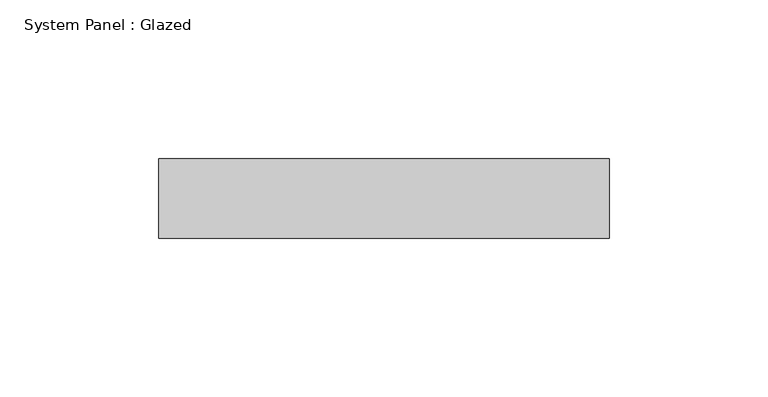
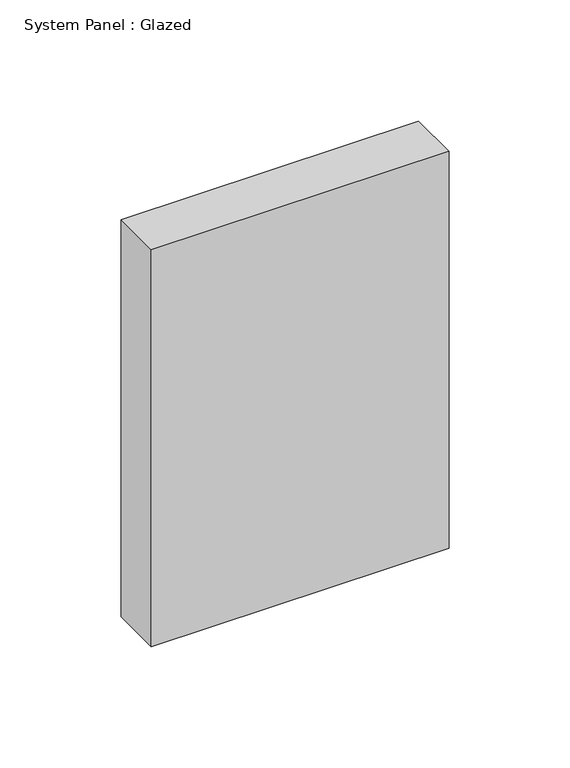
"""IFC4 building model written with IfcOpenShell, lengths in millimetres: plate geometry, System Panel : Glazed."""

import ifcopenshell
import ifcopenshell.guid

model = None  # the IFC model being written
_history = None  # IfcOwnerHistory: only IFC2X3 demands one
_inside = {}  # id of a spatial element -> (the spatial element, [elements in it])
_under = {}  # id of a project, library or spatial element -> (it, [spatial elements below it])
_declared = {}  # id of a project -> (the project, [libraries it declares])
_typed = {}  # id of a type object -> (the type object, [elements of that type])
_made_of = {}  # id of a material, layer set ... -> (it, [elements and type objects made of it])


def new_model(schema):
    """Start an empty IFC model of exactly this schema.

    Asked for "IFC4X3", IfcOpenShell would pick the latest addendum, in which some entities
    have other attributes; the version numbers below select the first issue.
    IFC2X3 requires an IfcOwnerHistory on every rooted entity: one is made here for all.
    """
    global model, _history
    if schema == "IFC4X3":
        model = ifcopenshell.file(schema_version=(4, 3, 0, 0))
    else:
        model = ifcopenshell.file(schema=schema)
    _inside.clear()
    _under.clear()
    _declared.clear()
    _typed.clear()
    _made_of.clear()
    _history = None
    if model.schema == "IFC2X3":
        org = make("IfcOrganization", Name="unknown")
        user = make(
            "IfcPersonAndOrganization",
            ThePerson=make("IfcPerson", FamilyName="unknown"),
            TheOrganization=org,
        )
        app = make(
            "IfcApplication",
            ApplicationDeveloper=org,
            Version="unknown",
            ApplicationFullName="unknown",
            ApplicationIdentifier="unknown",
        )
        _history = make(
            "IfcOwnerHistory",
            OwningUser=user,
            OwningApplication=app,
            ChangeAction="ADDED",
            CreationDate=0,
        )
    return model


def make(cls, **values):
    """One entity of the class cls with the attributes given. An attribute that is None is left unset."""
    return model.create_entity(
        cls, **{name: value for name, value in values.items() if value is not None}
    )


def rooted(cls, **values):
    """An entity with a GlobalId (a new one), such as an element, a storey or a relation."""
    return make(cls, GlobalId=ifcopenshell.guid.new(), OwnerHistory=_history, **values)


def si_unit(unit_type, name, prefix=None):
    """IfcSIUnit, for example si_unit("LENGTHUNIT", "METRE", prefix="MILLI")."""
    return make("IfcSIUnit", UnitType=unit_type, Prefix=prefix, Name=name)


def assignment(units):
    """IfcUnitAssignment: the units of a project."""
    return None if units is None else make("IfcUnitAssignment", Units=units)


def point(xyz):
    """IfcCartesianPoint."""
    return None if xyz is None else make("IfcCartesianPoint", Coordinates=xyz)


def direction(xyz):
    """IfcDirection."""
    return None if xyz is None else make("IfcDirection", DirectionRatios=xyz)


def frame(location, z_axis=None, x_axis=None):
    """IfcAxis2Placement3D, a coordinate frame: its origin and axes. An axis left out is left unset."""
    return make(
        "IfcAxis2Placement3D",
        Location=point(location),
        Axis=direction(z_axis),
        RefDirection=direction(x_axis),
    )


def origin():
    """The frame at (0, 0, 0) with its axes left unset."""
    return frame((0.0, 0.0, 0.0))


def origin_with_axes():
    """The frame at (0, 0, 0) with the z axis (0, 0, 1) and the x axis (1, 0, 0) written out."""
    return frame((0.0, 0.0, 0.0), z_axis=(0.0, 0.0, 1.0), x_axis=(1.0, 0.0, 0.0))


def place(relative_to, where):
    """IfcLocalPlacement: puts the frame where relative to a parent placement (None: the world)."""
    return make(
        "IfcLocalPlacement", PlacementRelTo=relative_to, RelativePlacement=where
    )


def context(
    kind, dimensions, precision=None, world=None, true_north=None, identifier=None
):
    """IfcGeometricRepresentationContext, for example the 3D "Model" context."""
    return make(
        "IfcGeometricRepresentationContext",
        ContextIdentifier=identifier,
        ContextType=kind,
        CoordinateSpaceDimension=dimensions,
        Precision=precision,
        WorldCoordinateSystem=world,
        TrueNorth=true_north,
    )


def project(units=None, contexts=None):
    """IfcProject with its units and contexts."""
    return rooted(
        "IfcProject",
        Name="project",
        RepresentationContexts=contexts,
        UnitsInContext=assignment(units),
    )


def spatial(cls, under=None, at=None, **own):
    """A site, building, storey or space (cls), placed at a placement, below another one or the project."""
    s = rooted(cls, ObjectPlacement=at, **own)
    if under is not None:
        _under.setdefault(under.id(), (under, []))[1].append(s)
    return s


def polyline(points):
    """IfcPolyline through the points."""
    return make("IfcPolyline", Points=[point(p) for p in points])


def outline(outer, holes=None, kind="AREA"):
    """IfcArbitraryClosedProfileDef: a profile drawn as a closed curve; with holes, ...WithVoids."""
    if holes is None:
        return make("IfcArbitraryClosedProfileDef", ProfileType=kind, OuterCurve=outer)
    return make(
        "IfcArbitraryProfileDefWithVoids",
        ProfileType=kind,
        OuterCurve=outer,
        InnerCurves=holes,
    )


def extrude(swept, where, along, depth):
    """IfcExtrudedAreaSolid: the profile swept, set in the frame where, extruded along a direction by depth."""
    return make(
        "IfcExtrudedAreaSolid",
        SweptArea=swept,
        Position=where,
        ExtrudedDirection=direction(along),
        Depth=depth,
    )


def shape(context_of_items, identifier, shape_type, items):
    """IfcShapeRepresentation: the items that make up one representation, for example the "Body"."""
    return make(
        "IfcShapeRepresentation",
        ContextOfItems=context_of_items,
        RepresentationIdentifier=identifier,
        RepresentationType=shape_type,
        Items=items,
    )


def source(mapping_origin, context_of_items, identifier, shape_type, items):
    """IfcRepresentationMap: a shape defined once, which mapped items show again and again."""
    return make(
        "IfcRepresentationMap",
        MappingOrigin=mapping_origin,
        MappedRepresentation=shape(context_of_items, identifier, shape_type, items),
    )


def transform(
    local_origin,
    x_axis=None,
    y_axis=None,
    z_axis=None,
    scale=None,
    scale2=None,
    scale3=None,
    uniform=True,
):
    """IfcCartesianTransformationOperator3D, or its non-uniform kind. x_axis, y_axis, z_axis: its Axis1, 2, 3."""
    if uniform:
        return make(
            "IfcCartesianTransformationOperator3D",
            Axis1=direction(x_axis),
            Axis2=direction(y_axis),
            LocalOrigin=point(local_origin),
            Scale=scale,
            Axis3=direction(z_axis),
        )
    return make(
        "IfcCartesianTransformationOperator3DnonUniform",
        Axis1=direction(x_axis),
        Axis2=direction(y_axis),
        LocalOrigin=point(local_origin),
        Scale=scale,
        Axis3=direction(z_axis),
        Scale2=scale2,
        Scale3=scale3,
    )


def mapped(mapping_source, mapping_target):
    """IfcMappedItem: shows the shape of a source again, moved by a transform."""
    return make(
        "IfcMappedItem", MappingSource=mapping_source, MappingTarget=mapping_target
    )


def made_of(thing, what):
    """Note that an element or type object is made of a material, layer set ...; save() writes the relation."""
    if what is not None:
        _made_of.setdefault(what.id(), (what, []))[1].append(thing)
    return thing


def element(
    cls,
    number,
    at=None,
    inside=None,
    cuts=None,
    type_object=None,
    material=None,
    context=None,
    identifier="Body",
    shape_type=None,
    held_by="IfcProductDefinitionShape",
    body=None,
    shapes=None,
    **own,
):
    """One element of the class cls, such as IfcWall. Its Tag is "e" and its number.

    at: its placement. inside: the storey or other place that contains it. cuts: it is an
    opening in that element (IfcRelVoidsElement). A single representation is given by context,
    identifier, shape_type and body (its items); several are given by shapes. held_by: the class
    of the entity that holds the representations. save() writes the other relations.
    """
    e = rooted(cls, Tag="e%d" % number, ObjectPlacement=at, **own)
    if body is not None:
        shapes = [shape(context, identifier, shape_type, body)]
    if shapes is not None:
        e.Representation = make(held_by, Representations=shapes)
    if inside is not None:
        _inside.setdefault(inside.id(), (inside, []))[1].append(e)
    if cuts is not None:
        rooted(
            "IfcRelVoidsElement", RelatingBuildingElement=cuts, RelatedOpeningElement=e
        )
    if type_object is not None:
        _typed.setdefault(type_object.id(), (type_object, []))[1].append(e)
    return made_of(e, material)


def aggregate(whole, parts):
    """IfcRelAggregates: a whole, such as a stair, and the parts it consists of."""
    return rooted("IfcRelAggregates", RelatingObject=whole, RelatedObjects=parts)


def save(model, path):
    """Write the relations noted so far, then the file.

    IfcRelAggregates (storeys below a building ...), IfcRelContainedInSpatialStructure (elements
    in a storey), IfcRelDefinesByType, IfcRelAssociatesMaterial and IfcRelDeclares: one each for
    every whole, place, type object, material and project.
    """
    for whole, parts in _under.values():
        aggregate(whole, parts)
    for where, things in _inside.values():
        rooted(
            "IfcRelContainedInSpatialStructure",
            RelatedElements=things,
            RelatingStructure=where,
        )
    for kind, things in _typed.values():
        rooted("IfcRelDefinesByType", RelatedObjects=things, RelatingType=kind)
    for what, things in _made_of.values():
        rooted("IfcRelAssociatesMaterial", RelatedObjects=things, RelatingMaterial=what)
    for by, libraries in _declared.values():
        rooted("IfcRelDeclares", RelatingContext=by, RelatedDefinitions=libraries)
    model.write(path)


def system_panel_glazed_de50ea70(model_context):
    return source(origin(), model_context, "Body", "SweptSolid", [
        extrude(outline(polyline([(70.9525426, 24.5), (-70.9525426, 24.5), (-70.9525426, 49.5), (70.9525426, 49.5), (70.9525426, 24.5)])), origin_with_axes(), (0.0, 0.0, 1.0), 200.0),
    ])


if __name__ == "__main__":
    model = new_model("IFC4")
    model_context = context("Model", 3, world=origin())
    ifc_project = project(units=[si_unit("LENGTHUNIT", "METRE", prefix="MILLI")], contexts=[model_context])
    site = spatial("IfcSite", under=ifc_project)
    building = spatial("IfcBuilding", under=site)
    placement = place(None, origin())
    system_panel_glazed_shape = system_panel_glazed_de50ea70(model_context)
    element("IfcPlate", 1, ObjectType="System Panel : Glazed", at=placement, inside=building, context=model_context, shape_type="MappedRepresentation", body=[
        mapped(system_panel_glazed_shape, transform((0.0, 0.0, 0.0), x_axis=(1.0, 0.0, 0.0), y_axis=(0.0, 1.0, 0.0), z_axis=(0.0, 0.0, 1.0))),
    ])
    save(model, "model.ifc")

# Revit data of these elements
# Element 1 (IfcPlate, "System Panel : Glazed")
#   Materials on its faces: "Glass"
# Materials
#   "Glass": class "Glass", colour RGB 218 227 224, transparency 0.85, Description = "Soda Lime Glass", Cost = 0
